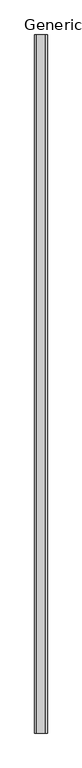
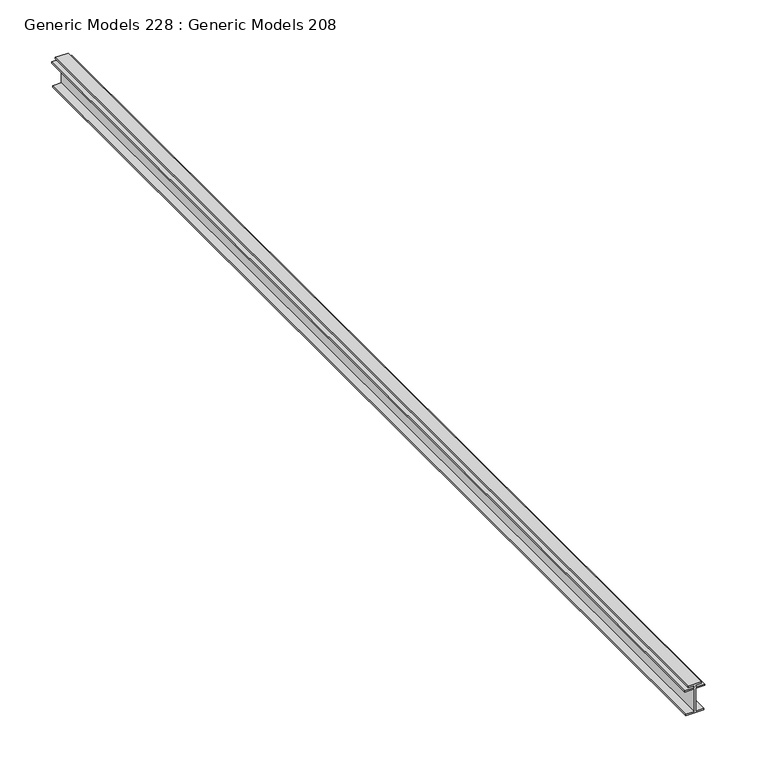
"""IFC4 building model written with IfcOpenShell, lengths in millimetres: proxy geometry, Generic Models 228 : Generic Models 208."""

from ifc_helpers import new_model, si_unit, frame, origin, place, context, project, spatial, polyline, outline, extrude, source, transform, mapped, element, save


def generic_models_228_generic_models_208_9bf69301(model_context):
    return source(origin(), model_context, "Body", "SweptSolid", [
        extrude(outline(polyline([(2164.159375, 54385.3792403), (2164.159375, 54395.6642176), (2137.4318993, 54395.6642176), (2137.4318993, 54386.2844915), (2135.8443993, 54386.2844915), (2135.8443993, 54406.3434243), (2137.4318993, 54406.3434243), (2137.4318993, 54397.2517176), (2164.159375, 54397.2517176), (2164.159375, 54407.4800364), (2165.746875, 54407.4800364), (2165.746875, 54397.2517176), (2168.128125, 54397.2517176), (2168.128125, 54403.6017176), (2169.715625, 54403.6017176), (2169.715625, 54389.0261981), (2168.128125, 54389.0261981), (2168.128125, 54395.6642176), (2165.746875, 54395.6642176), (2165.746875, 54385.3792403), (2164.159375, 54385.3792403)])), frame((0.0, -228.7033818, 0.0), z_axis=(0.0, 1.0, 0.0), x_axis=(0.0, 0.0, 1.0)), (0.0, 0.0, 1.0), 1219.2),
    ])


if __name__ == "__main__":
    model = new_model("IFC4")
    model_context = context("Model", 3, world=origin())
    ifc_project = project(units=[si_unit("LENGTHUNIT", "METRE", prefix="MILLI")], contexts=[model_context])
    site = spatial("IfcSite", under=ifc_project)
    building = spatial("IfcBuilding", under=site)
    placement = place(None, origin())
    generic_models_228_generic_models_208_shape = generic_models_228_generic_models_208_9bf69301(model_context)
    element("IfcBuildingElementProxy", 1, Name="Generic Models 228 : Generic Models 208", ObjectType="Generic Models 228 : Generic Models 208", at=placement, inside=building, context=model_context, shape_type="MappedRepresentation", body=[
        mapped(generic_models_228_generic_models_208_shape, transform((0.0, 0.0, 0.0), x_axis=(1.0, 0.0, 0.0), y_axis=(0.0, 1.0, 0.0), z_axis=(0.0, 0.0, 1.0))),
    ])
    save(model, "model.ifc")
